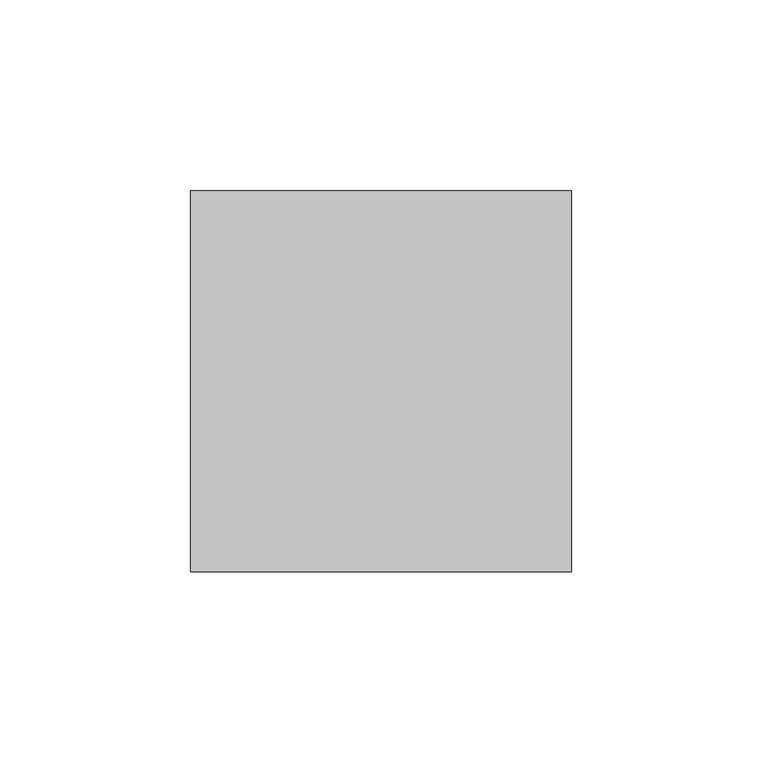
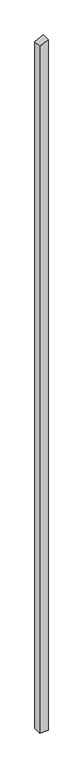
"""IFC4 building model written with IfcOpenShell, lengths in millimetres: column geometry, Holzstütze 159506 : Holzstütze 159506."""

from ifc_helpers import new_model, si_unit, frame, origin, place, context, project, spatial, polyline, outline, extrude, source, transform, mapped, element, save


def column_c64e92fe(model_context):
    return source(origin(), model_context, "Body", "SweptSolid", [
        extrude(outline(polyline([(-500.0, 161027.7593015), (-500.0, 161127.7593015), (8297.1942973, 161127.7593015), (8246.2417524, 161027.7593015), (-500.0, 161027.7593015)])), frame((0.0, 26981.9343946, 0.0), z_axis=(0.0, 1.0, 0.0), x_axis=(0.0, 0.0, 1.0)), (0.0, 0.0, 1.0), 100.0),
    ])


if __name__ == "__main__":
    model = new_model("IFC4")
    model_context = context("Model", 3, world=origin())
    ifc_project = project(units=[si_unit("LENGTHUNIT", "METRE", prefix="MILLI")], contexts=[model_context])
    site = spatial("IfcSite", under=ifc_project)
    building = spatial("IfcBuilding", under=site)
    placement = place(None, origin())
    column_shape = column_c64e92fe(model_context)
    element("IfcColumn", 1, ObjectType="Holzstütze 159506 : Holzstütze 159506", at=placement, inside=building, context=model_context, shape_type="MappedRepresentation", body=[
        mapped(column_shape, transform((0.0, 0.0, 0.0), x_axis=(1.0, 0.0, 0.0), y_axis=(0.0, 1.0, 0.0), z_axis=(0.0, 0.0, 1.0))),
    ])
    save(model, "model.ifc")

# Revit data of these elements
# Type "Holzstütze 159506 : Holzstütze 159506"
#   Abrechnungsart = "m"
#   Allright_Bauteil_ID = "0152St 0000143549"
#   Bezeichnung = "Holzstütze"
#   Codetext = "ST-HOLZ\\"
#   Gewerk = "Zimmer- und Holzbauarbeiten"
#   Material = "Holz"
#   Objektname = "Stütze"
#   NameOverride = "Holzstütze"
#   Reference = "Holzstütze"
#   Status = "NEW"
#   ThermalTransmittance = 0.0000 BTU/(h·ft²·°F)
#   Roll = 0.00°
#   Slope = 0.00°
#   2D Interaktion = yes
#   IsExternal = yes
#   LoadBearing = yes
# Element 1 (IfcColumn, "Holzstütze 159506 : Holzstütze 159506")
#   Materials on its faces: "holzschalung"
# Materials
#   "holzschalung": class "Unassigned", colour RGB 128 128 128, transparency 0
